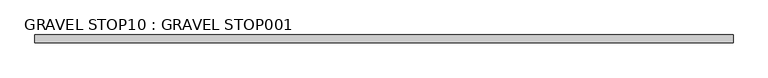
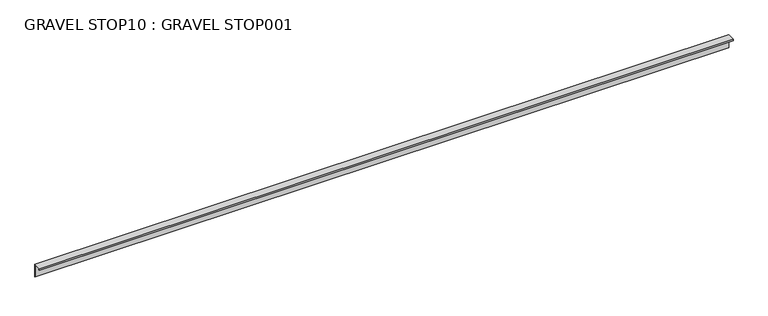
"""IFC4 building model written with IfcOpenShell, lengths in millimetres: proxy geometry, GRAVEL STOP10 : GRAVEL STOP001."""

from ifc_helpers import new_model, si_unit, frame, origin, place, context, project, spatial, polyline, outline, extrude, source, transform, mapped, element, save


def gravel_stop10_gravel_stop001_c600786e(model_context):
    return source(origin(), model_context, "Body", "SweptSolid", [
        extrude(outline(polyline([(-5562.4629675, 40210.7296087), (-5582.1479675, 40210.7296087), (-5582.1479675, 40208.5198087), (-5580.4155111, 40208.5198087), (-5580.4155111, 40207.2498087), (-5583.4179675, 40207.2498087), (-5583.4179675, 40211.9996087), (-5561.1929675, 40211.9996087), (-5561.1929675, 40173.8996087), (-5562.4629675, 40173.8996087), (-5562.4629675, 40210.7296087)])), frame((12382.7678845, 0.0, 0.0), z_axis=(1.0, 0.0, 0.0), x_axis=(0.0, 1.0, 0.0)), (0.0, 0.0, 1.0), 2000.25),
    ])


if __name__ == "__main__":
    model = new_model("IFC4")
    model_context = context("Model", 3, world=origin())
    ifc_project = project(units=[si_unit("LENGTHUNIT", "METRE", prefix="MILLI")], contexts=[model_context])
    site = spatial("IfcSite", under=ifc_project)
    building = spatial("IfcBuilding", under=site)
    placement = place(None, origin())
    gravel_stop10_gravel_stop001_shape = gravel_stop10_gravel_stop001_c600786e(model_context)
    element("IfcBuildingElementProxy", 1, Name="GRAVEL STOP10 : GRAVEL STOP001", ObjectType="GRAVEL STOP10 : GRAVEL STOP001", at=placement, inside=building, context=model_context, shape_type="MappedRepresentation", body=[
        mapped(gravel_stop10_gravel_stop001_shape, transform((0.0, 0.0, 0.0), x_axis=(1.0, 0.0, 0.0), y_axis=(0.0, 1.0, 0.0), z_axis=(0.0, 0.0, 1.0))),
    ])
    save(model, "model.ifc")

# Revit data of these elements
# Type "GRAVEL STOP10 : GRAVEL STOP001"
#   NameOverride = "GRAVEL STOP001"
# Element 1 (IfcBuildingElementProxy, "GRAVEL STOP10 : GRAVEL STOP001")
#   Materials on its faces: "COPPER STUCCO J BEAD"
# Materials
#   "COPPER STUCCO J BEAD": class "Unassigned", colour RGB 251 232 155, transparency 0, Cost = 0
